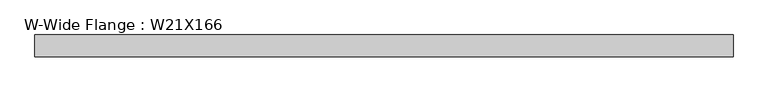
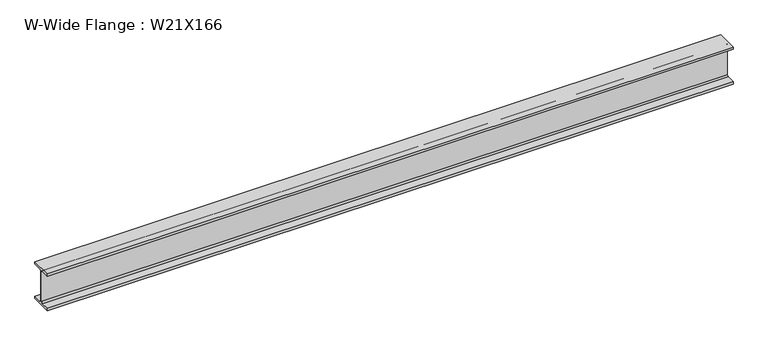
"""IFC4 building model written with IfcOpenShell, lengths in millimetres: beam geometry, W-Wide Flange : W21X166."""

from ifc_helpers import new_model, si_unit, point, frame, frame_2d, origin, place, context, project, spatial, polyline, circle_curve, trimmed, segment, composite_curve, outline, extrude, source, transform, mapped, element, save


def w_wide_flange_w21x166_19d43a63(model_context):
    return source(origin(), model_context, "Body", "SweptSolid", [
        extrude(outline(composite_curve([segment(polyline([(157.48, -251.206), (157.48, -285.75), (-157.48, -285.75), (-157.48, -251.206), (-32.131, -251.206)]), True, "CONTINUOUS"), segment(trimmed(circle_curve(frame_2d((-32.131, -228.6)), 22.606), [point((-32.131, -251.206))], [point((-9.525, -228.6))], True, "CARTESIAN"), True, "CONTINUOUS"), segment(polyline([(-9.525, -228.6), (-9.525, 228.6)]), True, "CONTINUOUS"), segment(trimmed(circle_curve(frame_2d((-32.131, 228.6)), 22.606), [point((-9.525, 228.6))], [point((-32.131, 251.206))], True, "CARTESIAN"), True, "CONTINUOUS"), segment(polyline([(-32.131, 251.206), (-157.48, 251.206), (-157.48, 285.75), (157.48, 285.75), (157.48, 251.206), (32.131, 251.206)]), True, "CONTINUOUS"), segment(trimmed(circle_curve(frame_2d((32.131, 228.6)), 22.606), [point((32.131, 251.206))], [point((9.525, 228.6))], True, "CARTESIAN"), True, "CONTINUOUS"), segment(polyline([(9.525, 228.6), (9.525, -228.6)]), True, "CONTINUOUS"), segment(trimmed(circle_curve(frame_2d((32.131, -228.6)), 22.606), [point((9.525, -228.6))], [point((32.131, -251.206))], True, "CARTESIAN"), True, "CONTINUOUS"), segment(polyline([(32.131, -251.206), (157.48, -251.206)]), True, "CONTINUOUS")], self_intersect=False)), frame((-5139.310137, 0.0, 0.0), z_axis=(1.0, 0.0, 0.0), x_axis=(0.0, 1.0, 0.0)), (0.0, 0.0, 1.0), 10050.7427444),
    ])


if __name__ == "__main__":
    model = new_model("IFC4")
    model_context = context("Model", 3, world=origin())
    ifc_project = project(units=[si_unit("LENGTHUNIT", "METRE", prefix="MILLI")], contexts=[model_context])
    site = spatial("IfcSite", under=ifc_project)
    building = spatial("IfcBuilding", under=site)
    placement = place(None, origin())
    w_wide_flange_w21x166_shape = w_wide_flange_w21x166_19d43a63(model_context)
    element("IfcBeam", 1, ObjectType="W-Wide Flange : W21X166", at=placement, inside=building, context=model_context, shape_type="MappedRepresentation", body=[
        mapped(w_wide_flange_w21x166_shape, transform((0.0, 0.0, 0.0), x_axis=(1.0, 0.0, 0.0), y_axis=(0.0, 1.0, 0.0), z_axis=(0.0, 0.0, 1.0))),
    ])
    save(model, "model.ifc")

# Revit data of these elements
# Type "W-Wide Flange : W21X166"
#   Assembly Code = "B10"
#   W = 166
#   Length [instance default] = 5' - 0"
#   bf = 1' - 0.4"
#   d = 1' - 10 1/2"
#   k = 0' - 2 1/4"
#   k2 = 0' - 0.89"
#   tf = 0' - 1.36"
#   tw = 0' - 0 3/4"
#   A = 0.338889 SF
#   Structural Material [instance default] = Steel ASTM A992
# Element 1 (IfcBeam, "W-Wide Flange : W21X166")
#   Structural Material = Steel
#   Materials on its faces: "Steel"
# Materials
#   "Steel ASTM A992": class "Metal", colour RGB 199 199 199, transparency 0, Description = "Structural steel 50ksi", Cost = 0
#   "Steel": class "Metal", colour RGB 118 118 114, transparency 0, Description = "Steel, mill finish", Cost = 0
